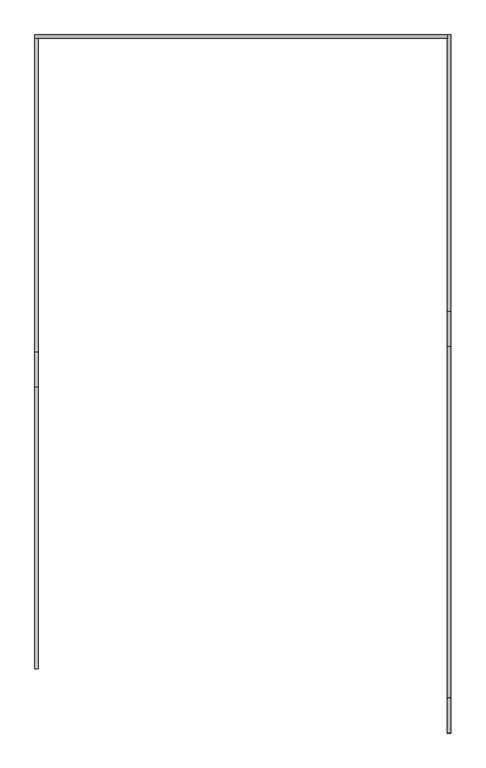
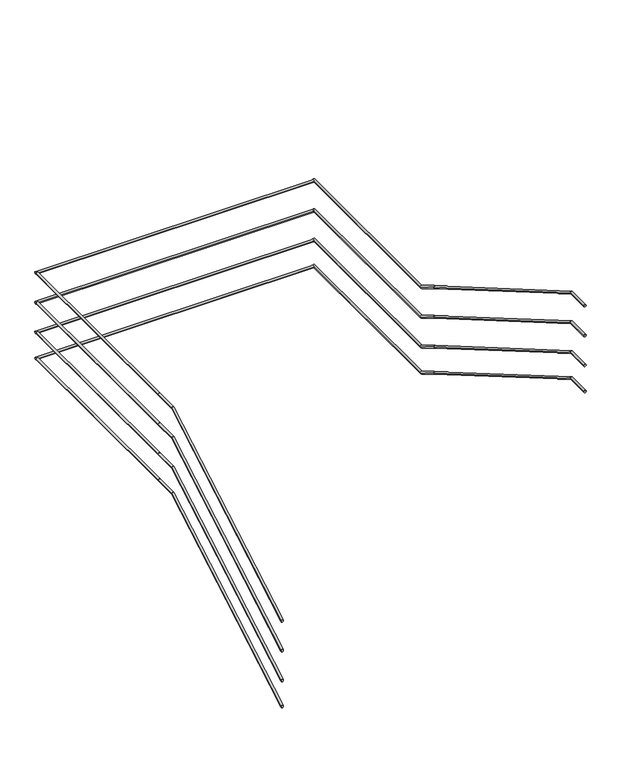
"""IFC4 building model written with IfcOpenShell, lengths in millimetres: railing geometry."""

from ifc_helpers import new_model, si_unit, frame, origin, place, context, project, spatial, circle_curve, ellipse_curve, source, transform, mapped, element, save
from ifc_brep_helpers import plane_surface, cylinder_surface, advanced_brep


def railing_c3b53c4a(model_context):
    return source(origin(), model_context, "Body", "AdvancedBrep", [
        advanced_brep(
        [(51115.4, 12129.5208589, 7307.5963084), (51085.4, 12129.5208589, 7307.5963084), (51115.4, 14533.576096, 8709.9618634), (51085.4, 14533.576096, 8709.9618634), (51115.4, 14829.5208589, 8709.9618634), (51085.4, 14829.5208589, 8709.9618634)],
        [
            (0, 1, ellipse_curve(frame((51100.4, 12129.5208589, 7307.5963084), z_axis=(0.0, -1.0, 0.0), x_axis=(0.0, 0.0, -1.0)), 17.365555, 15.0)),
            (1, 0, ellipse_curve(frame((51100.4, 12129.5208589, 7307.5963084), z_axis=(0.0, -1.0, 0.0), x_axis=(0.0, 0.0, -1.0)), 17.365555, 15.0)),
            (0, 2),
            (2, 3, ellipse_curve(frame((51100.4, 14533.576096, 8709.9618634), z_axis=(0.0, -0.9653442134540491, -0.26097997921446625), x_axis=(0.0, 0.2609799792144657, -0.9653442134540494)), 15.5384989, 15.0)),
            (3, 1),
            (3, 2, ellipse_curve(frame((51100.4, 14533.576096, 8709.9618634), z_axis=(0.0, -0.9653442134540491, -0.26097997921446625), x_axis=(0.0, 0.2609799792144657, -0.9653442134540494)), 15.5384989, 15.0)),
            (4, 5, circle_curve(frame((51100.4, 14829.5208589, 8709.9618634), z_axis=(0.0, 1.0, 0.0), x_axis=(-1.0, 0.0, 0.0)), 15.0)),
            (5, 4, circle_curve(frame((51100.4, 14829.5208589, 8709.9618634), z_axis=(0.0, 1.0, 0.0), x_axis=(-1.0, 0.0, 0.0)), 15.0)),
            (2, 4),
            (5, 3),
        ],
        [
            plane_surface(frame((51100.4, 12129.5208589, 7324.9618634), z_axis=(0.0, -1.0, 0.0), x_axis=(0.0, 0.0, 1.0))),
            cylinder_surface(frame((51100.4, 12137.0789243, 7312.0051799), z_axis=(0.0, -0.8637789008984336, -0.5038710255240861), x_axis=(-1.0, 0.0, 0.0)), 15.0),
            plane_surface(frame((51100.4, 14829.5208589, 8724.9618634), z_axis=(0.0, 1.0, 0.0), x_axis=(0.0, 0.0, 1.0))),
            cylinder_surface(frame((51100.4, 14529.5208589, 8709.9618634), z_axis=(0.0, -1.0, 0.0), x_axis=(-1.0, 0.0, 0.0)), 15.0),
        ],
        [
            (0, [[1, 2]]),
            (1, [[-1, 3, 4, 5]]),
            (1, [[-2, -5, 6, -3]]),
            (2, [[7, 8]]),
            (3, [[-4, 9, -8, 10]]),
            (3, [[-6, -10, -7, -9]]),
        ],
    ),
        advanced_brep(
        [(51115.4, 14829.5208589, 8709.9618634), (51085.4, 14829.5208589, 8709.9618634), (51115.4, 17509.1208589, 8709.9618634), (51085.4, 17509.1208589, 8709.9618634)],
        [
            (0, 1, circle_curve(frame((51100.4, 14829.5208589, 8709.9618634), z_axis=(0.0, -1.0, 0.0), x_axis=(-1.0, 0.0, 0.0)), 15.0)),
            (1, 0, circle_curve(frame((51100.4, 14829.5208589, 8709.9618634), z_axis=(0.0, -1.0, 0.0), x_axis=(-1.0, 0.0, 0.0)), 15.0)),
            (2, 3, circle_curve(frame((51100.4, 17509.1208589, 8709.9618634), z_axis=(0.0, 1.0, 0.0), x_axis=(-1.0, 0.0, 0.0)), 15.0)),
            (3, 2, circle_curve(frame((51100.4, 17509.1208589, 8709.9618634), z_axis=(0.0, 1.0, 0.0), x_axis=(-1.0, 0.0, 0.0)), 15.0)),
            (0, 2),
            (3, 1),
        ],
        [
            plane_surface(frame((51100.4, 14829.5208589, 8724.9618634), z_axis=(0.0, -1.0, 0.0), x_axis=(0.0, 0.0, 1.0))),
            plane_surface(frame((51100.4, 17509.1208589, 8724.9618634), z_axis=(0.0, 1.0, 0.0), x_axis=(0.0, 0.0, 1.0))),
            cylinder_surface(frame((51100.4, 14829.5208589, 8709.9618634), z_axis=(0.0, -1.0, 0.0), x_axis=(-1.0, 0.0, 0.0)), 15.0),
        ],
        [
            (0, [[1, 2]]),
            (1, [[3, 4]]),
            (2, [[-1, 5, -4, 6]]),
            (2, [[-2, -6, -3, -5]]),
        ],
    ),
        advanced_brep(
        [(51085.4, 17509.1208589, 8709.9618634), (51085.4, 17539.1208589, 8709.9618634), (54609.6, 17509.1208589, 8709.9618634), (54609.6, 17539.1208589, 8709.9618634)],
        [
            (0, 1, circle_curve(frame((51085.4, 17524.1208589, 8709.9618634), z_axis=(-1.0, 0.0, 0.0), x_axis=(0.0, 1.0, 0.0)), 15.0)),
            (1, 0, circle_curve(frame((51085.4, 17524.1208589, 8709.9618634), z_axis=(-1.0, 0.0, 0.0), x_axis=(0.0, 1.0, 0.0)), 15.0)),
            (2, 3, circle_curve(frame((54609.6, 17524.1208589, 8709.9618634), z_axis=(1.0, 0.0, 0.0), x_axis=(0.0, 1.0, 0.0)), 15.0)),
            (3, 2, circle_curve(frame((54609.6, 17524.1208589, 8709.9618634), z_axis=(1.0, 0.0, 0.0), x_axis=(0.0, 1.0, 0.0)), 15.0)),
            (0, 2),
            (3, 1),
        ],
        [
            plane_surface(frame((51085.4, 17524.1208589, 8724.9618634), z_axis=(-1.0, 0.0, 0.0), x_axis=(0.0, 1.0, 0.0))),
            plane_surface(frame((54609.6, 17524.1208589, 8724.9618634), z_axis=(1.0, 0.0, 0.0), x_axis=(0.0, 1.0, 0.0))),
            cylinder_surface(frame((51085.4, 17524.1208589, 8709.9618634), z_axis=(-1.0, 0.0, 0.0), x_axis=(0.0, 1.0, 0.0)), 15.0),
        ],
        [
            (0, [[1, 2]]),
            (1, [[3, 4]]),
            (2, [[-1, 5, -4, 6]]),
            (2, [[-2, -6, -3, -5]]),
        ],
    ),
        advanced_brep(
        [(54609.6, 17539.1208589, 8709.9618634), (54639.6, 17539.1208589, 8709.9618634), (54609.6, 15175.4656218, 8709.9618634), (54639.6, 15175.4656218, 8709.9618634), (54609.6, 14879.5208589, 8882.5963084), (54639.6, 14879.5208589, 8882.5963084)],
        [
            (0, 1, circle_curve(frame((54624.6, 17539.1208589, 8709.9618634), z_axis=(0.0, 1.0, 0.0), x_axis=(1.0, 0.0, 0.0)), 15.0)),
            (1, 0, circle_curve(frame((54624.6, 17539.1208589, 8709.9618634), z_axis=(0.0, 1.0, 0.0), x_axis=(1.0, 0.0, 0.0)), 15.0)),
            (0, 2),
            (2, 3, ellipse_curve(frame((54624.6, 15175.4656218, 8709.9618634), z_axis=(0.0, 0.9653442134540493, -0.26097997921446586), x_axis=(0.0, 0.2609799792144653, 0.9653442134540493)), 15.5384989, 15.0)),
            (3, 1),
            (3, 2, ellipse_curve(frame((54624.6, 15175.4656218, 8709.9618634), z_axis=(0.0, 0.9653442134540493, -0.26097997921446586), x_axis=(0.0, 0.2609799792144653, 0.9653442134540493)), 15.5384989, 15.0)),
            (4, 5, ellipse_curve(frame((54624.6, 14879.5208589, 8882.5963084), z_axis=(0.0, -1.0, 0.0), x_axis=(0.0, 0.0, -1.0)), 17.365555, 15.0)),
            (5, 4, ellipse_curve(frame((54624.6, 14879.5208589, 8882.5963084), z_axis=(0.0, -1.0, 0.0), x_axis=(0.0, 0.0, -1.0)), 17.365555, 15.0)),
            (2, 4),
            (5, 3),
        ],
        [
            plane_surface(frame((54624.6, 17539.1208589, 8724.9618634), z_axis=(0.0, 1.0, 0.0), x_axis=(0.0, 0.0, -1.0))),
            cylinder_surface(frame((54624.6, 17539.1208589, 8709.9618634), z_axis=(0.0, 1.0, 0.0), x_axis=(1.0, 0.0, 0.0)), 15.0),
            plane_surface(frame((54624.6, 14879.5208589, 8899.9618634), z_axis=(0.0, -1.0, 0.0), x_axis=(0.0, 0.0, -1.0))),
            cylinder_surface(frame((54624.6, 15171.9627935, 8712.0051799), z_axis=(0.0, 0.8637789008984339, -0.5038710255240854), x_axis=(1.0, 0.0, 0.0)), 15.0),
        ],
        [
            (0, [[1, 2]]),
            (1, [[-1, 3, 4, 5]]),
            (1, [[-2, -5, 6, -3]]),
            (2, [[7, 8]]),
            (3, [[-4, 9, -8, 10]]),
            (3, [[-6, -10, -7, -9]]),
        ],
    ),
        advanced_brep(
        [(54609.6, 14879.5208589, 8882.5963084), (54639.6, 14879.5208589, 8882.5963084), (54609.6, 11875.4656218, 10634.9618634), (54639.6, 11875.4656218, 10634.9618634), (54609.6, 11579.5208589, 10634.9618634), (54639.6, 11579.5208589, 10634.9618634)],
        [
            (0, 1, ellipse_curve(frame((54624.6, 14879.5208589, 8882.5963084), z_axis=(0.0, 1.0, 0.0), x_axis=(0.0, 0.0, -1.0)), 17.365555, 15.0)),
            (1, 0, ellipse_curve(frame((54624.6, 14879.5208589, 8882.5963084), z_axis=(0.0, 1.0, 0.0), x_axis=(0.0, 0.0, -1.0)), 17.365555, 15.0)),
            (0, 2),
            (2, 3, ellipse_curve(frame((54624.6, 11875.4656218, 10634.9618634), z_axis=(0.0, 0.9653442134540491, -0.26097997921446625), x_axis=(0.0, -0.2609799792144661, -0.9653442134540492)), 15.5384989, 15.0)),
            (3, 1),
            (3, 2, ellipse_curve(frame((54624.6, 11875.4656218, 10634.9618634), z_axis=(0.0, 0.9653442134540491, -0.26097997921446625), x_axis=(0.0, -0.2609799792144661, -0.9653442134540492)), 15.5384989, 15.0)),
            (4, 5, circle_curve(frame((54624.6, 11579.5208589, 10634.9618634), z_axis=(0.0, -1.0, 0.0), x_axis=(1.0, 0.0, 0.0)), 15.0)),
            (5, 4, circle_curve(frame((54624.6, 11579.5208589, 10634.9618634), z_axis=(0.0, -1.0, 0.0), x_axis=(1.0, 0.0, 0.0)), 15.0)),
            (2, 4),
            (5, 3),
        ],
        [
            plane_surface(frame((54624.6, 14879.5208589, 8899.9618634), z_axis=(0.0, 1.0, 0.0), x_axis=(0.0, 0.0, -1.0))),
            cylinder_surface(frame((54624.6, 14871.9627935, 8887.0051799), z_axis=(0.0, 0.8637789008984335, -0.5038710255240861), x_axis=(1.0, 0.0, 0.0)), 15.0),
            plane_surface(frame((54624.6, 11579.5208589, 10649.9618634), z_axis=(0.0, -1.0, 0.0), x_axis=(0.0, 0.0, -1.0))),
            cylinder_surface(frame((54624.6, 11879.5208589, 10634.9618634), z_axis=(0.0, 1.0, 0.0), x_axis=(1.0, 0.0, 0.0)), 15.0),
        ],
        [
            (0, [[1, 2]]),
            (1, [[-1, 3, 4, 5]]),
            (1, [[-2, -5, 6, -3]]),
            (2, [[7, 8]]),
            (3, [[-4, 9, -8, 10]]),
            (3, [[-6, -10, -7, -9]]),
        ],
    ),
        advanced_brep(
        [(51115.4, 12129.5208589, 6507.5963084), (51085.4, 12129.5208589, 6507.5963084), (51115.4, 14533.576096, 7909.9618634), (51085.4, 14533.576096, 7909.9618634), (51115.4, 14829.5208589, 7909.9618634), (51085.4, 14829.5208589, 7909.9618634)],
        [
            (0, 1, ellipse_curve(frame((51100.4, 12129.5208589, 6507.5963084), z_axis=(0.0, -1.0, 0.0), x_axis=(0.0, 0.0, -1.0)), 17.365555, 15.0)),
            (1, 0, ellipse_curve(frame((51100.4, 12129.5208589, 6507.5963084), z_axis=(0.0, -1.0, 0.0), x_axis=(0.0, 0.0, -1.0)), 17.365555, 15.0)),
            (0, 2),
            (2, 3, ellipse_curve(frame((51100.4, 14533.576096, 7909.9618634), z_axis=(0.0, -0.9653442134540491, -0.26097997921446625), x_axis=(0.0, 0.2609799792144657, -0.9653442134540494)), 15.5384989, 15.0)),
            (3, 1),
            (3, 2, ellipse_curve(frame((51100.4, 14533.576096, 7909.9618634), z_axis=(0.0, -0.9653442134540491, -0.26097997921446625), x_axis=(0.0, 0.2609799792144657, -0.9653442134540494)), 15.5384989, 15.0)),
            (4, 5, circle_curve(frame((51100.4, 14829.5208589, 7909.9618634), z_axis=(0.0, 1.0, 0.0), x_axis=(-1.0, 0.0, 0.0)), 15.0)),
            (5, 4, circle_curve(frame((51100.4, 14829.5208589, 7909.9618634), z_axis=(0.0, 1.0, 0.0), x_axis=(-1.0, 0.0, 0.0)), 15.0)),
            (2, 4),
            (5, 3),
        ],
        [
            plane_surface(frame((51100.4, 12129.5208589, 6524.9618634), z_axis=(0.0, -1.0, 0.0), x_axis=(0.0, 0.0, 1.0))),
            cylinder_surface(frame((51100.4, 12137.0789243, 6512.0051799), z_axis=(0.0, -0.8637789008984336, -0.5038710255240861), x_axis=(-1.0, 0.0, 0.0)), 15.0),
            plane_surface(frame((51100.4, 14829.5208589, 7924.9618634), z_axis=(0.0, 1.0, 0.0), x_axis=(0.0, 0.0, 1.0))),
            cylinder_surface(frame((51100.4, 14529.5208589, 7909.9618634), z_axis=(0.0, -1.0, 0.0), x_axis=(-1.0, 0.0, 0.0)), 15.0),
        ],
        [
            (0, [[1, 2]]),
            (1, [[-1, 3, 4, 5]]),
            (1, [[-2, -5, 6, -3]]),
            (2, [[7, 8]]),
            (3, [[-4, 9, -8, 10]]),
            (3, [[-6, -10, -7, -9]]),
        ],
    ),
        advanced_brep(
        [(51115.4, 14829.5208589, 7909.9618634), (51085.4, 14829.5208589, 7909.9618634), (51115.4, 17509.1208589, 7909.9618634), (51085.4, 17509.1208589, 7909.9618634)],
        [
            (0, 1, circle_curve(frame((51100.4, 14829.5208589, 7909.9618634), z_axis=(0.0, -1.0, 0.0), x_axis=(-1.0, 0.0, 0.0)), 15.0)),
            (1, 0, circle_curve(frame((51100.4, 14829.5208589, 7909.9618634), z_axis=(0.0, -1.0, 0.0), x_axis=(-1.0, 0.0, 0.0)), 15.0)),
            (2, 3, circle_curve(frame((51100.4, 17509.1208589, 7909.9618634), z_axis=(0.0, 1.0, 0.0), x_axis=(-1.0, 0.0, 0.0)), 15.0)),
            (3, 2, circle_curve(frame((51100.4, 17509.1208589, 7909.9618634), z_axis=(0.0, 1.0, 0.0), x_axis=(-1.0, 0.0, 0.0)), 15.0)),
            (0, 2),
            (3, 1),
        ],
        [
            plane_surface(frame((51100.4, 14829.5208589, 7924.9618634), z_axis=(0.0, -1.0, 0.0), x_axis=(0.0, 0.0, 1.0))),
            plane_surface(frame((51100.4, 17509.1208589, 7924.9618634), z_axis=(0.0, 1.0, 0.0), x_axis=(0.0, 0.0, 1.0))),
            cylinder_surface(frame((51100.4, 14829.5208589, 7909.9618634), z_axis=(0.0, -1.0, 0.0), x_axis=(-1.0, 0.0, 0.0)), 15.0),
        ],
        [
            (0, [[1, 2]]),
            (1, [[3, 4]]),
            (2, [[-1, 5, -4, 6]]),
            (2, [[-2, -6, -3, -5]]),
        ],
    ),
        advanced_brep(
        [(51085.4, 17509.1208589, 7909.9618634), (51085.4, 17539.1208589, 7909.9618634), (54609.6, 17509.1208589, 7909.9618634), (54609.6, 17539.1208589, 7909.9618634)],
        [
            (0, 1, circle_curve(frame((51085.4, 17524.1208589, 7909.9618634), z_axis=(-1.0, 0.0, 0.0), x_axis=(0.0, 1.0, 0.0)), 15.0)),
            (1, 0, circle_curve(frame((51085.4, 17524.1208589, 7909.9618634), z_axis=(-1.0, 0.0, 0.0), x_axis=(0.0, 1.0, 0.0)), 15.0)),
            (2, 3, circle_curve(frame((54609.6, 17524.1208589, 7909.9618634), z_axis=(1.0, 0.0, 0.0), x_axis=(0.0, 1.0, 0.0)), 15.0)),
            (3, 2, circle_curve(frame((54609.6, 17524.1208589, 7909.9618634), z_axis=(1.0, 0.0, 0.0), x_axis=(0.0, 1.0, 0.0)), 15.0)),
            (0, 2),
            (3, 1),
        ],
        [
            plane_surface(frame((51085.4, 17524.1208589, 7924.9618634), z_axis=(-1.0, 0.0, 0.0), x_axis=(0.0, 1.0, 0.0))),
            plane_surface(frame((54609.6, 17524.1208589, 7924.9618634), z_axis=(1.0, 0.0, 0.0), x_axis=(0.0, 1.0, 0.0))),
            cylinder_surface(frame((51085.4, 17524.1208589, 7909.9618634), z_axis=(-1.0, 0.0, 0.0), x_axis=(0.0, 1.0, 0.0)), 15.0),
        ],
        [
            (0, [[1, 2]]),
            (1, [[3, 4]]),
            (2, [[-1, 5, -4, 6]]),
            (2, [[-2, -6, -3, -5]]),
        ],
    ),
        advanced_brep(
        [(54609.6, 17539.1208589, 7909.9618634), (54639.6, 17539.1208589, 7909.9618634), (54609.6, 15175.4656218, 7909.9618634), (54639.6, 15175.4656218, 7909.9618634), (54609.6, 14879.5208589, 8082.5963084), (54639.6, 14879.5208589, 8082.5963084)],
        [
            (0, 1, circle_curve(frame((54624.6, 17539.1208589, 7909.9618634), z_axis=(0.0, 1.0, 0.0), x_axis=(1.0, 0.0, 0.0)), 15.0)),
            (1, 0, circle_curve(frame((54624.6, 17539.1208589, 7909.9618634), z_axis=(0.0, 1.0, 0.0), x_axis=(1.0, 0.0, 0.0)), 15.0)),
            (0, 2),
            (2, 3, ellipse_curve(frame((54624.6, 15175.4656218, 7909.9618634), z_axis=(0.0, 0.9653442134540493, -0.26097997921446586), x_axis=(0.0, 0.2609799792144653, 0.9653442134540493)), 15.5384989, 15.0)),
            (3, 1),
            (3, 2, ellipse_curve(frame((54624.6, 15175.4656218, 7909.9618634), z_axis=(0.0, 0.9653442134540493, -0.26097997921446586), x_axis=(0.0, 0.2609799792144653, 0.9653442134540493)), 15.5384989, 15.0)),
            (4, 5, ellipse_curve(frame((54624.6, 14879.5208589, 8082.5963084), z_axis=(0.0, -1.0, 0.0), x_axis=(0.0, 0.0, -1.0)), 17.365555, 15.0)),
            (5, 4, ellipse_curve(frame((54624.6, 14879.5208589, 8082.5963084), z_axis=(0.0, -1.0, 0.0), x_axis=(0.0, 0.0, -1.0)), 17.365555, 15.0)),
            (2, 4),
            (5, 3),
        ],
        [
            plane_surface(frame((54624.6, 17539.1208589, 7924.9618634), z_axis=(0.0, 1.0, 0.0), x_axis=(0.0, 0.0, -1.0))),
            cylinder_surface(frame((54624.6, 17539.1208589, 7909.9618634), z_axis=(0.0, 1.0, 0.0), x_axis=(1.0, 0.0, 0.0)), 15.0),
            plane_surface(frame((54624.6, 14879.5208589, 8099.9618634), z_axis=(0.0, -1.0, 0.0), x_axis=(0.0, 0.0, -1.0))),
            cylinder_surface(frame((54624.6, 15171.9627935, 7912.0051799), z_axis=(0.0, 0.8637789008984339, -0.5038710255240854), x_axis=(1.0, 0.0, 0.0)), 15.0),
        ],
        [
            (0, [[1, 2]]),
            (1, [[-1, 3, 4, 5]]),
            (1, [[-2, -5, 6, -3]]),
            (2, [[7, 8]]),
            (3, [[-4, 9, -8, 10]]),
            (3, [[-6, -10, -7, -9]]),
        ],
    ),
        advanced_brep(
        [(54609.6, 14879.5208589, 8082.5963084), (54639.6, 14879.5208589, 8082.5963084), (54609.6, 11875.4656218, 9834.9618634), (54639.6, 11875.4656218, 9834.9618634), (54609.6, 11579.5208589, 9834.9618634), (54639.6, 11579.5208589, 9834.9618634)],
        [
            (0, 1, ellipse_curve(frame((54624.6, 14879.5208589, 8082.5963084), z_axis=(0.0, 1.0, 0.0), x_axis=(0.0, 0.0, -1.0)), 17.365555, 15.0)),
            (1, 0, ellipse_curve(frame((54624.6, 14879.5208589, 8082.5963084), z_axis=(0.0, 1.0, 0.0), x_axis=(0.0, 0.0, -1.0)), 17.365555, 15.0)),
            (0, 2),
            (2, 3, ellipse_curve(frame((54624.6, 11875.4656218, 9834.9618634), z_axis=(0.0, 0.9653442134540491, -0.26097997921446625), x_axis=(0.0, -0.2609799792144661, -0.9653442134540492)), 15.5384989, 15.0)),
            (3, 1),
            (3, 2, ellipse_curve(frame((54624.6, 11875.4656218, 9834.9618634), z_axis=(0.0, 0.9653442134540491, -0.26097997921446625), x_axis=(0.0, -0.2609799792144661, -0.9653442134540492)), 15.5384989, 15.0)),
            (4, 5, circle_curve(frame((54624.6, 11579.5208589, 9834.9618634), z_axis=(0.0, -1.0, 0.0), x_axis=(1.0, 0.0, 0.0)), 15.0)),
            (5, 4, circle_curve(frame((54624.6, 11579.5208589, 9834.9618634), z_axis=(0.0, -1.0, 0.0), x_axis=(1.0, 0.0, 0.0)), 15.0)),
            (2, 4),
            (5, 3),
        ],
        [
            plane_surface(frame((54624.6, 14879.5208589, 8099.9618634), z_axis=(0.0, 1.0, 0.0), x_axis=(0.0, 0.0, -1.0))),
            cylinder_surface(frame((54624.6, 14871.9627935, 8087.0051799), z_axis=(0.0, 0.8637789008984335, -0.5038710255240861), x_axis=(1.0, 0.0, 0.0)), 15.0),
            plane_surface(frame((54624.6, 11579.5208589, 9849.9618634), z_axis=(0.0, -1.0, 0.0), x_axis=(0.0, 0.0, -1.0))),
            cylinder_surface(frame((54624.6, 11879.5208589, 9834.9618634), z_axis=(0.0, 1.0, 0.0), x_axis=(1.0, 0.0, 0.0)), 15.0),
        ],
        [
            (0, [[1, 2]]),
            (1, [[-1, 3, 4, 5]]),
            (1, [[-2, -5, 6, -3]]),
            (2, [[7, 8]]),
            (3, [[-4, 9, -8, 10]]),
            (3, [[-6, -10, -7, -9]]),
        ],
    ),
        advanced_brep(
        [(51115.4, 12129.5208589, 6907.5963084), (51085.4, 12129.5208589, 6907.5963084), (51115.4, 14533.576096, 8309.9618634), (51085.4, 14533.576096, 8309.9618634), (51115.4, 14829.5208589, 8309.9618634), (51085.4, 14829.5208589, 8309.9618634)],
        [
            (0, 1, ellipse_curve(frame((51100.4, 12129.5208589, 6907.5963084), z_axis=(0.0, -1.0, 0.0), x_axis=(0.0, 0.0, -1.0)), 17.365555, 15.0)),
            (1, 0, ellipse_curve(frame((51100.4, 12129.5208589, 6907.5963084), z_axis=(0.0, -1.0, 0.0), x_axis=(0.0, 0.0, -1.0)), 17.365555, 15.0)),
            (0, 2),
            (2, 3, ellipse_curve(frame((51100.4, 14533.576096, 8309.9618634), z_axis=(0.0, -0.9653442134540491, -0.26097997921446625), x_axis=(0.0, 0.2609799792144657, -0.9653442134540494)), 15.5384989, 15.0)),
            (3, 1),
            (3, 2, ellipse_curve(frame((51100.4, 14533.576096, 8309.9618634), z_axis=(0.0, -0.9653442134540491, -0.26097997921446625), x_axis=(0.0, 0.2609799792144657, -0.9653442134540494)), 15.5384989, 15.0)),
            (4, 5, circle_curve(frame((51100.4, 14829.5208589, 8309.9618634), z_axis=(0.0, 1.0, 0.0), x_axis=(-1.0, 0.0, 0.0)), 15.0)),
            (5, 4, circle_curve(frame((51100.4, 14829.5208589, 8309.9618634), z_axis=(0.0, 1.0, 0.0), x_axis=(-1.0, 0.0, 0.0)), 15.0)),
            (2, 4),
            (5, 3),
        ],
        [
            plane_surface(frame((51100.4, 12129.5208589, 6924.9618634), z_axis=(0.0, -1.0, 0.0), x_axis=(0.0, 0.0, 1.0))),
            cylinder_surface(frame((51100.4, 12137.0789243, 6912.0051799), z_axis=(0.0, -0.8637789008984336, -0.5038710255240861), x_axis=(-1.0, 0.0, 0.0)), 15.0),
            plane_surface(frame((51100.4, 14829.5208589, 8324.9618634), z_axis=(0.0, 1.0, 0.0), x_axis=(0.0, 0.0, 1.0))),
            cylinder_surface(frame((51100.4, 14529.5208589, 8309.9618634), z_axis=(0.0, -1.0, 0.0), x_axis=(-1.0, 0.0, 0.0)), 15.0),
        ],
        [
            (0, [[1, 2]]),
            (1, [[-1, 3, 4, 5]]),
            (1, [[-2, -5, 6, -3]]),
            (2, [[7, 8]]),
            (3, [[-4, 9, -8, 10]]),
            (3, [[-6, -10, -7, -9]]),
        ],
    ),
        advanced_brep(
        [(51115.4, 14829.5208589, 8309.9618634), (51085.4, 14829.5208589, 8309.9618634), (51115.4, 17509.1208589, 8309.9618634), (51085.4, 17509.1208589, 8309.9618634)],
        [
            (0, 1, circle_curve(frame((51100.4, 14829.5208589, 8309.9618634), z_axis=(0.0, -1.0, 0.0), x_axis=(-1.0, 0.0, 0.0)), 15.0)),
            (1, 0, circle_curve(frame((51100.4, 14829.5208589, 8309.9618634), z_axis=(0.0, -1.0, 0.0), x_axis=(-1.0, 0.0, 0.0)), 15.0)),
            (2, 3, circle_curve(frame((51100.4, 17509.1208589, 8309.9618634), z_axis=(0.0, 1.0, 0.0), x_axis=(-1.0, 0.0, 0.0)), 15.0)),
            (3, 2, circle_curve(frame((51100.4, 17509.1208589, 8309.9618634), z_axis=(0.0, 1.0, 0.0), x_axis=(-1.0, 0.0, 0.0)), 15.0)),
            (0, 2),
            (3, 1),
        ],
        [
            plane_surface(frame((51100.4, 14829.5208589, 8324.9618634), z_axis=(0.0, -1.0, 0.0), x_axis=(0.0, 0.0, 1.0))),
            plane_surface(frame((51100.4, 17509.1208589, 8324.9618634), z_axis=(0.0, 1.0, 0.0), x_axis=(0.0, 0.0, 1.0))),
            cylinder_surface(frame((51100.4, 14829.5208589, 8309.9618634), z_axis=(0.0, -1.0, 0.0), x_axis=(-1.0, 0.0, 0.0)), 15.0),
        ],
        [
            (0, [[1, 2]]),
            (1, [[3, 4]]),
            (2, [[-1, 5, -4, 6]]),
            (2, [[-2, -6, -3, -5]]),
        ],
    ),
        advanced_brep(
        [(51085.4, 17509.1208589, 8309.9618634), (51085.4, 17539.1208589, 8309.9618634), (54609.6, 17509.1208589, 8309.9618634), (54609.6, 17539.1208589, 8309.9618634)],
        [
            (0, 1, circle_curve(frame((51085.4, 17524.1208589, 8309.9618634), z_axis=(-1.0, 0.0, 0.0), x_axis=(0.0, 1.0, 0.0)), 15.0)),
            (1, 0, circle_curve(frame((51085.4, 17524.1208589, 8309.9618634), z_axis=(-1.0, 0.0, 0.0), x_axis=(0.0, 1.0, 0.0)), 15.0)),
            (2, 3, circle_curve(frame((54609.6, 17524.1208589, 8309.9618634), z_axis=(1.0, 0.0, 0.0), x_axis=(0.0, 1.0, 0.0)), 15.0)),
            (3, 2, circle_curve(frame((54609.6, 17524.1208589, 8309.9618634), z_axis=(1.0, 0.0, 0.0), x_axis=(0.0, 1.0, 0.0)), 15.0)),
            (0, 2),
            (3, 1),
        ],
        [
            plane_surface(frame((51085.4, 17524.1208589, 8324.9618634), z_axis=(-1.0, 0.0, 0.0), x_axis=(0.0, 1.0, 0.0))),
            plane_surface(frame((54609.6, 17524.1208589, 8324.9618634), z_axis=(1.0, 0.0, 0.0), x_axis=(0.0, 1.0, 0.0))),
            cylinder_surface(frame((51085.4, 17524.1208589, 8309.9618634), z_axis=(-1.0, 0.0, 0.0), x_axis=(0.0, 1.0, 0.0)), 15.0),
        ],
        [
            (0, [[1, 2]]),
            (1, [[3, 4]]),
            (2, [[-1, 5, -4, 6]]),
            (2, [[-2, -6, -3, -5]]),
        ],
    ),
        advanced_brep(
        [(54609.6, 17539.1208589, 8309.9618634), (54639.6, 17539.1208589, 8309.9618634), (54609.6, 15175.4656218, 8309.9618634), (54639.6, 15175.4656218, 8309.9618634), (54609.6, 14879.5208589, 8482.5963084), (54639.6, 14879.5208589, 8482.5963084)],
        [
            (0, 1, circle_curve(frame((54624.6, 17539.1208589, 8309.9618634), z_axis=(0.0, 1.0, 0.0), x_axis=(1.0, 0.0, 0.0)), 15.0)),
            (1, 0, circle_curve(frame((54624.6, 17539.1208589, 8309.9618634), z_axis=(0.0, 1.0, 0.0), x_axis=(1.0, 0.0, 0.0)), 15.0)),
            (0, 2),
            (2, 3, ellipse_curve(frame((54624.6, 15175.4656218, 8309.9618634), z_axis=(0.0, 0.9653442134540493, -0.26097997921446586), x_axis=(0.0, 0.2609799792144653, 0.9653442134540493)), 15.5384989, 15.0)),
            (3, 1),
            (3, 2, ellipse_curve(frame((54624.6, 15175.4656218, 8309.9618634), z_axis=(0.0, 0.9653442134540493, -0.26097997921446586), x_axis=(0.0, 0.2609799792144653, 0.9653442134540493)), 15.5384989, 15.0)),
            (4, 5, ellipse_curve(frame((54624.6, 14879.5208589, 8482.5963084), z_axis=(0.0, -1.0, 0.0), x_axis=(0.0, 0.0, -1.0)), 17.365555, 15.0)),
            (5, 4, ellipse_curve(frame((54624.6, 14879.5208589, 8482.5963084), z_axis=(0.0, -1.0, 0.0), x_axis=(0.0, 0.0, -1.0)), 17.365555, 15.0)),
            (2, 4),
            (5, 3),
        ],
        [
            plane_surface(frame((54624.6, 17539.1208589, 8324.9618634), z_axis=(0.0, 1.0, 0.0), x_axis=(0.0, 0.0, -1.0))),
            cylinder_surface(frame((54624.6, 17539.1208589, 8309.9618634), z_axis=(0.0, 1.0, 0.0), x_axis=(1.0, 0.0, 0.0)), 15.0),
            plane_surface(frame((54624.6, 14879.5208589, 8499.9618634), z_axis=(0.0, -1.0, 0.0), x_axis=(0.0, 0.0, -1.0))),
            cylinder_surface(frame((54624.6, 15171.9627935, 8312.0051799), z_axis=(0.0, 0.8637789008984339, -0.5038710255240854), x_axis=(1.0, 0.0, 0.0)), 15.0),
        ],
        [
            (0, [[1, 2]]),
            (1, [[-1, 3, 4, 5]]),
            (1, [[-2, -5, 6, -3]]),
            (2, [[7, 8]]),
            (3, [[-4, 9, -8, 10]]),
            (3, [[-6, -10, -7, -9]]),
        ],
    ),
        advanced_brep(
        [(54609.6, 14879.5208589, 8482.5963084), (54639.6, 14879.5208589, 8482.5963084), (54609.6, 11875.4656218, 10234.9618634), (54639.6, 11875.4656218, 10234.9618634), (54609.6, 11579.5208589, 10234.9618634), (54639.6, 11579.5208589, 10234.9618634)],
        [
            (0, 1, ellipse_curve(frame((54624.6, 14879.5208589, 8482.5963084), z_axis=(0.0, 1.0, 0.0), x_axis=(0.0, 0.0, -1.0)), 17.365555, 15.0)),
            (1, 0, ellipse_curve(frame((54624.6, 14879.5208589, 8482.5963084), z_axis=(0.0, 1.0, 0.0), x_axis=(0.0, 0.0, -1.0)), 17.365555, 15.0)),
            (0, 2),
            (2, 3, ellipse_curve(frame((54624.6, 11875.4656218, 10234.9618634), z_axis=(0.0, 0.9653442134540491, -0.26097997921446625), x_axis=(0.0, -0.2609799792144661, -0.9653442134540492)), 15.5384989, 15.0)),
            (3, 1),
            (3, 2, ellipse_curve(frame((54624.6, 11875.4656218, 10234.9618634), z_axis=(0.0, 0.9653442134540491, -0.26097997921446625), x_axis=(0.0, -0.2609799792144661, -0.9653442134540492)), 15.5384989, 15.0)),
            (4, 5, circle_curve(frame((54624.6, 11579.5208589, 10234.9618634), z_axis=(0.0, -1.0, 0.0), x_axis=(1.0, 0.0, 0.0)), 15.0)),
            (5, 4, circle_curve(frame((54624.6, 11579.5208589, 10234.9618634), z_axis=(0.0, -1.0, 0.0), x_axis=(1.0, 0.0, 0.0)), 15.0)),
            (2, 4),
            (5, 3),
        ],
        [
            plane_surface(frame((54624.6, 14879.5208589, 8499.9618634), z_axis=(0.0, 1.0, 0.0), x_axis=(0.0, 0.0, -1.0))),
            cylinder_surface(frame((54624.6, 14871.9627935, 8487.0051799), z_axis=(0.0, 0.8637789008984335, -0.5038710255240861), x_axis=(1.0, 0.0, 0.0)), 15.0),
            plane_surface(frame((54624.6, 11579.5208589, 10249.9618634), z_axis=(0.0, -1.0, 0.0), x_axis=(0.0, 0.0, -1.0))),
            cylinder_surface(frame((54624.6, 11879.5208589, 10234.9618634), z_axis=(0.0, 1.0, 0.0), x_axis=(1.0, 0.0, 0.0)), 15.0),
        ],
        [
            (0, [[1, 2]]),
            (1, [[-1, 3, 4, 5]]),
            (1, [[-2, -5, 6, -3]]),
            (2, [[7, 8]]),
            (3, [[-4, 9, -8, 10]]),
            (3, [[-6, -10, -7, -9]]),
        ],
    ),
        advanced_brep(
        [(51115.4, 12129.5208589, 6157.5963084), (51085.4, 12129.5208589, 6157.5963084), (51115.4, 14533.576096, 7559.9618634), (51085.4, 14533.576096, 7559.9618634), (51115.4, 14829.5208589, 7559.9618634), (51085.4, 14829.5208589, 7559.9618634)],
        [
            (0, 1, ellipse_curve(frame((51100.4, 12129.5208589, 6157.5963084), z_axis=(0.0, -1.0, 0.0), x_axis=(0.0, 0.0, -1.0)), 17.365555, 15.0)),
            (1, 0, ellipse_curve(frame((51100.4, 12129.5208589, 6157.5963084), z_axis=(0.0, -1.0, 0.0), x_axis=(0.0, 0.0, -1.0)), 17.365555, 15.0)),
            (0, 2),
            (2, 3, ellipse_curve(frame((51100.4, 14533.576096, 7559.9618634), z_axis=(0.0, -0.9653442134540491, -0.26097997921446625), x_axis=(0.0, 0.2609799792144657, -0.9653442134540494)), 15.5384989, 15.0)),
            (3, 1),
            (3, 2, ellipse_curve(frame((51100.4, 14533.576096, 7559.9618634), z_axis=(0.0, -0.9653442134540491, -0.26097997921446625), x_axis=(0.0, 0.2609799792144657, -0.9653442134540494)), 15.5384989, 15.0)),
            (4, 5, circle_curve(frame((51100.4, 14829.5208589, 7559.9618634), z_axis=(0.0, 1.0, 0.0), x_axis=(-1.0, 0.0, 0.0)), 15.0)),
            (5, 4, circle_curve(frame((51100.4, 14829.5208589, 7559.9618634), z_axis=(0.0, 1.0, 0.0), x_axis=(-1.0, 0.0, 0.0)), 15.0)),
            (2, 4),
            (5, 3),
        ],
        [
            plane_surface(frame((51100.4, 12129.5208589, 6174.9618634), z_axis=(0.0, -1.0, 0.0), x_axis=(0.0, 0.0, 1.0))),
            cylinder_surface(frame((51100.4, 12137.0789243, 6162.0051799), z_axis=(0.0, -0.8637789008984336, -0.5038710255240861), x_axis=(-1.0, 0.0, 0.0)), 15.0),
            plane_surface(frame((51100.4, 14829.5208589, 7574.9618634), z_axis=(0.0, 1.0, 0.0), x_axis=(0.0, 0.0, 1.0))),
            cylinder_surface(frame((51100.4, 14529.5208589, 7559.9618634), z_axis=(0.0, -1.0, 0.0), x_axis=(-1.0, 0.0, 0.0)), 15.0),
        ],
        [
            (0, [[1, 2]]),
            (1, [[-1, 3, 4, 5]]),
            (1, [[-2, -5, 6, -3]]),
            (2, [[7, 8]]),
            (3, [[-4, 9, -8, 10]]),
            (3, [[-6, -10, -7, -9]]),
        ],
    ),
        advanced_brep(
        [(51115.4, 14829.5208589, 7559.9618634), (51085.4, 14829.5208589, 7559.9618634), (51115.4, 17509.1208589, 7559.9618634), (51085.4, 17509.1208589, 7559.9618634)],
        [
            (0, 1, circle_curve(frame((51100.4, 14829.5208589, 7559.9618634), z_axis=(0.0, -1.0, 0.0), x_axis=(-1.0, 0.0, 0.0)), 15.0)),
            (1, 0, circle_curve(frame((51100.4, 14829.5208589, 7559.9618634), z_axis=(0.0, -1.0, 0.0), x_axis=(-1.0, 0.0, 0.0)), 15.0)),
            (2, 3, circle_curve(frame((51100.4, 17509.1208589, 7559.9618634), z_axis=(0.0, 1.0, 0.0), x_axis=(-1.0, 0.0, 0.0)), 15.0)),
            (3, 2, circle_curve(frame((51100.4, 17509.1208589, 7559.9618634), z_axis=(0.0, 1.0, 0.0), x_axis=(-1.0, 0.0, 0.0)), 15.0)),
            (0, 2),
            (3, 1),
        ],
        [
            plane_surface(frame((51100.4, 14829.5208589, 7574.9618634), z_axis=(0.0, -1.0, 0.0), x_axis=(0.0, 0.0, 1.0))),
            plane_surface(frame((51100.4, 17509.1208589, 7574.9618634), z_axis=(0.0, 1.0, 0.0), x_axis=(0.0, 0.0, 1.0))),
            cylinder_surface(frame((51100.4, 14829.5208589, 7559.9618634), z_axis=(0.0, -1.0, 0.0), x_axis=(-1.0, 0.0, 0.0)), 15.0),
        ],
        [
            (0, [[1, 2]]),
            (1, [[3, 4]]),
            (2, [[-1, 5, -4, 6]]),
            (2, [[-2, -6, -3, -5]]),
        ],
    ),
        advanced_brep(
        [(51085.4, 17509.1208589, 7559.9618634), (51085.4, 17539.1208589, 7559.9618634), (54609.6, 17509.1208589, 7559.9618634), (54609.6, 17539.1208589, 7559.9618634)],
        [
            (0, 1, circle_curve(frame((51085.4, 17524.1208589, 7559.9618634), z_axis=(-1.0, 0.0, 0.0), x_axis=(0.0, 1.0, 0.0)), 15.0)),
            (1, 0, circle_curve(frame((51085.4, 17524.1208589, 7559.9618634), z_axis=(-1.0, 0.0, 0.0), x_axis=(0.0, 1.0, 0.0)), 15.0)),
            (2, 3, circle_curve(frame((54609.6, 17524.1208589, 7559.9618634), z_axis=(1.0, 0.0, 0.0), x_axis=(0.0, 1.0, 0.0)), 15.0)),
            (3, 2, circle_curve(frame((54609.6, 17524.1208589, 7559.9618634), z_axis=(1.0, 0.0, 0.0), x_axis=(0.0, 1.0, 0.0)), 15.0)),
            (0, 2),
            (3, 1),
        ],
        [
            plane_surface(frame((51085.4, 17524.1208589, 7574.9618634), z_axis=(-1.0, 0.0, 0.0), x_axis=(0.0, 1.0, 0.0))),
            plane_surface(frame((54609.6, 17524.1208589, 7574.9618634), z_axis=(1.0, 0.0, 0.0), x_axis=(0.0, 1.0, 0.0))),
            cylinder_surface(frame((51085.4, 17524.1208589, 7559.9618634), z_axis=(-1.0, 0.0, 0.0), x_axis=(0.0, 1.0, 0.0)), 15.0),
        ],
        [
            (0, [[1, 2]]),
            (1, [[3, 4]]),
            (2, [[-1, 5, -4, 6]]),
            (2, [[-2, -6, -3, -5]]),
        ],
    ),
        advanced_brep(
        [(54609.6, 17539.1208589, 7559.9618634), (54639.6, 17539.1208589, 7559.9618634), (54609.6, 15175.4656218, 7559.9618634), (54639.6, 15175.4656218, 7559.9618634), (54609.6, 14879.5208589, 7732.5963084), (54639.6, 14879.5208589, 7732.5963084)],
        [
            (0, 1, circle_curve(frame((54624.6, 17539.1208589, 7559.9618634), z_axis=(0.0, 1.0, 0.0), x_axis=(1.0, 0.0, 0.0)), 15.0)),
            (1, 0, circle_curve(frame((54624.6, 17539.1208589, 7559.9618634), z_axis=(0.0, 1.0, 0.0), x_axis=(1.0, 0.0, 0.0)), 15.0)),
            (0, 2),
            (2, 3, ellipse_curve(frame((54624.6, 15175.4656218, 7559.9618634), z_axis=(0.0, 0.9653442134540493, -0.26097997921446586), x_axis=(0.0, 0.2609799792144653, 0.9653442134540493)), 15.5384989, 15.0)),
            (3, 1),
            (3, 2, ellipse_curve(frame((54624.6, 15175.4656218, 7559.9618634), z_axis=(0.0, 0.9653442134540493, -0.26097997921446586), x_axis=(0.0, 0.2609799792144653, 0.9653442134540493)), 15.5384989, 15.0)),
            (4, 5, ellipse_curve(frame((54624.6, 14879.5208589, 7732.5963084), z_axis=(0.0, -1.0, 0.0), x_axis=(0.0, 0.0, -1.0)), 17.365555, 15.0)),
            (5, 4, ellipse_curve(frame((54624.6, 14879.5208589, 7732.5963084), z_axis=(0.0, -1.0, 0.0), x_axis=(0.0, 0.0, -1.0)), 17.365555, 15.0)),
            (2, 4),
            (5, 3),
        ],
        [
            plane_surface(frame((54624.6, 17539.1208589, 7574.9618634), z_axis=(0.0, 1.0, 0.0), x_axis=(0.0, 0.0, -1.0))),
            cylinder_surface(frame((54624.6, 17539.1208589, 7559.9618634), z_axis=(0.0, 1.0, 0.0), x_axis=(1.0, 0.0, 0.0)), 15.0),
            plane_surface(frame((54624.6, 14879.5208589, 7749.9618634), z_axis=(0.0, -1.0, 0.0), x_axis=(0.0, 0.0, -1.0))),
            cylinder_surface(frame((54624.6, 15171.9627935, 7562.0051799), z_axis=(0.0, 0.8637789008984339, -0.5038710255240854), x_axis=(1.0, 0.0, 0.0)), 15.0),
        ],
        [
            (0, [[1, 2]]),
            (1, [[-1, 3, 4, 5]]),
            (1, [[-2, -5, 6, -3]]),
            (2, [[7, 8]]),
            (3, [[-4, 9, -8, 10]]),
            (3, [[-6, -10, -7, -9]]),
        ],
    ),
        advanced_brep(
        [(54609.6, 14879.5208589, 7732.5963084), (54639.6, 14879.5208589, 7732.5963084), (54609.6, 11875.4656218, 9484.9618634), (54639.6, 11875.4656218, 9484.9618634), (54609.6, 11579.5208589, 9484.9618634), (54639.6, 11579.5208589, 9484.9618634)],
        [
            (0, 1, ellipse_curve(frame((54624.6, 14879.5208589, 7732.5963084), z_axis=(0.0, 1.0, 0.0), x_axis=(0.0, 0.0, -1.0)), 17.365555, 15.0)),
            (1, 0, ellipse_curve(frame((54624.6, 14879.5208589, 7732.5963084), z_axis=(0.0, 1.0, 0.0), x_axis=(0.0, 0.0, -1.0)), 17.365555, 15.0)),
            (0, 2),
            (2, 3, ellipse_curve(frame((54624.6, 11875.4656218, 9484.9618634), z_axis=(0.0, 0.9653442134540491, -0.26097997921446625), x_axis=(0.0, -0.2609799792144661, -0.9653442134540492)), 15.5384989, 15.0)),
            (3, 1),
            (3, 2, ellipse_curve(frame((54624.6, 11875.4656218, 9484.9618634), z_axis=(0.0, 0.9653442134540491, -0.26097997921446625), x_axis=(0.0, -0.2609799792144661, -0.9653442134540492)), 15.5384989, 15.0)),
            (4, 5, circle_curve(frame((54624.6, 11579.5208589, 9484.9618634), z_axis=(0.0, -1.0, 0.0), x_axis=(1.0, 0.0, 0.0)), 15.0)),
            (5, 4, circle_curve(frame((54624.6, 11579.5208589, 9484.9618634), z_axis=(0.0, -1.0, 0.0), x_axis=(1.0, 0.0, 0.0)), 15.0)),
            (2, 4),
            (5, 3),
        ],
        [
            plane_surface(frame((54624.6, 14879.5208589, 7749.9618634), z_axis=(0.0, 1.0, 0.0), x_axis=(0.0, 0.0, -1.0))),
            cylinder_surface(frame((54624.6, 14871.9627935, 7737.0051799), z_axis=(0.0, 0.8637789008984335, -0.5038710255240861), x_axis=(1.0, 0.0, 0.0)), 15.0),
            plane_surface(frame((54624.6, 11579.5208589, 9499.9618634), z_axis=(0.0, -1.0, 0.0), x_axis=(0.0, 0.0, -1.0))),
            cylinder_surface(frame((54624.6, 11879.5208589, 9484.9618634), z_axis=(0.0, 1.0, 0.0), x_axis=(1.0, 0.0, 0.0)), 15.0),
        ],
        [
            (0, [[1, 2]]),
            (1, [[-1, 3, 4, 5]]),
            (1, [[-2, -5, 6, -3]]),
            (2, [[7, 8]]),
            (3, [[-4, 9, -8, 10]]),
            (3, [[-6, -10, -7, -9]]),
        ],
    ),
    ])


if __name__ == "__main__":
    model = new_model("IFC4")
    model_context = context("Model", 3, world=origin())
    ifc_project = project(units=[si_unit("LENGTHUNIT", "METRE", prefix="MILLI")], contexts=[model_context])
    site = spatial("IfcSite", under=ifc_project)
    building = spatial("IfcBuilding", under=site)
    placement = place(None, origin())
    railing_shape = railing_c3b53c4a(model_context)
    element("IfcRailing", 1, at=placement, inside=building, context=model_context, shape_type="MappedRepresentation", body=[
        mapped(railing_shape, transform((0.0, 0.0, 0.0), x_axis=(1.0, 0.0, 0.0), y_axis=(0.0, 1.0, 0.0), z_axis=(0.0, 0.0, 1.0))),
    ])
    save(model, "model.ifc")
